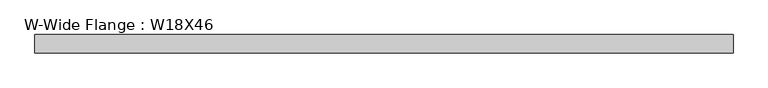
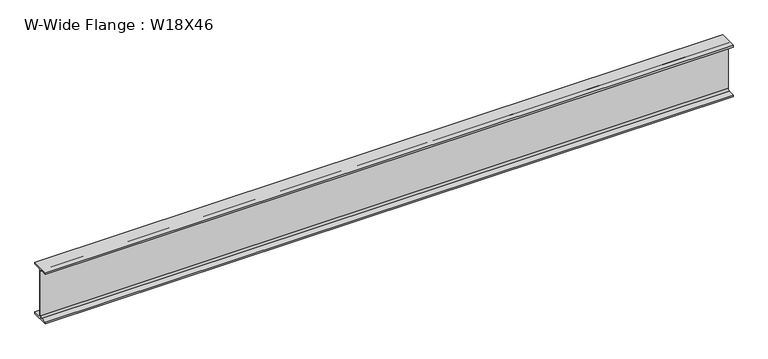
"""IFC4 building model written with IfcOpenShell, lengths in millimetres: beam geometry, W-Wide Flange : W18X46."""

from ifc_helpers import new_model, si_unit, point, frame, frame_2d, origin, place, context, project, spatial, polyline, circle_curve, trimmed, segment, composite_curve, outline, extrude, source, transform, mapped, element, save


def w_wide_flange_w18x46_ab9c9dab(model_context):
    return source(origin(), model_context, "Body", "SweptSolid", [
        extrude(outline(composite_curve([segment(polyline([(76.962, -214.503), (76.962, -229.87), (-76.962, -229.87), (-76.962, -214.503), (-20.955, -214.503)]), True, "CONTINUOUS"), segment(trimmed(circle_curve(frame_2d((-20.955, -198.12)), 16.383), [point((-20.955, -214.503))], [point((-4.572, -198.12))], True, "CARTESIAN"), True, "CONTINUOUS"), segment(polyline([(-4.572, -198.12), (-4.572, 198.12)]), True, "CONTINUOUS"), segment(trimmed(circle_curve(frame_2d((-20.955, 198.12)), 16.383), [point((-4.572, 198.12))], [point((-20.955, 214.503))], True, "CARTESIAN"), True, "CONTINUOUS"), segment(polyline([(-20.955, 214.503), (-76.962, 214.503), (-76.962, 229.87), (76.962, 229.87), (76.962, 214.503), (20.955, 214.503)]), True, "CONTINUOUS"), segment(trimmed(circle_curve(frame_2d((20.955, 198.12)), 16.383), [point((20.955, 214.503))], [point((4.572, 198.12))], True, "CARTESIAN"), True, "CONTINUOUS"), segment(polyline([(4.572, 198.12), (4.572, -198.12)]), True, "CONTINUOUS"), segment(trimmed(circle_curve(frame_2d((20.955, -198.12)), 16.383), [point((4.572, -198.12))], [point((20.955, -214.503))], True, "CARTESIAN"), True, "CONTINUOUS"), segment(polyline([(20.955, -214.503), (76.962, -214.503)]), True, "CONTINUOUS")], self_intersect=False)), frame((-2908.3, 0.0, 0.0), z_axis=(1.0, 0.0, 0.0), x_axis=(0.0, 1.0, 0.0)), (0.0, 0.0, 1.0), 5816.6),
    ])


if __name__ == "__main__":
    model = new_model("IFC4")
    model_context = context("Model", 3, world=origin())
    ifc_project = project(units=[si_unit("LENGTHUNIT", "METRE", prefix="MILLI")], contexts=[model_context])
    site = spatial("IfcSite", under=ifc_project)
    building = spatial("IfcBuilding", under=site)
    placement = place(None, origin())
    w_wide_flange_w18x46_shape = w_wide_flange_w18x46_ab9c9dab(model_context)
    element("IfcBeam", 1, ObjectType="W-Wide Flange : W18X46", at=placement, inside=building, context=model_context, shape_type="MappedRepresentation", body=[
        mapped(w_wide_flange_w18x46_shape, transform((0.0, 0.0, 0.0), x_axis=(1.0, 0.0, 0.0), y_axis=(0.0, 1.0, 0.0), z_axis=(0.0, 0.0, 1.0))),
    ])
    save(model, "model.ifc")

# Revit data of these elements
# Type "W-Wide Flange : W18X46"
#   Assembly Code = "B10"
#   W = 46
#   Length [instance default] = 5' - 0"
#   bf = 0' - 6.06"
#   d = 1' - 6.1"
#   k = 0' - 1 1/4"
#   k2 = 0' - 0.645"
#   tf = 0' - 0.605"
#   tw = 0' - 0.36"
#   A = 0.09375 SF
#   Structural Material [instance default] = Steel ASTM A992
# Element 1 (IfcBeam, "W-Wide Flange : W18X46")
#   Materials on its faces: "Steel ASTM A992"
# Materials
#   "Steel ASTM A992": class "Metal", colour RGB 199 199 199, transparency 0, Description = "Structural steel 50ksi", Cost = 0
